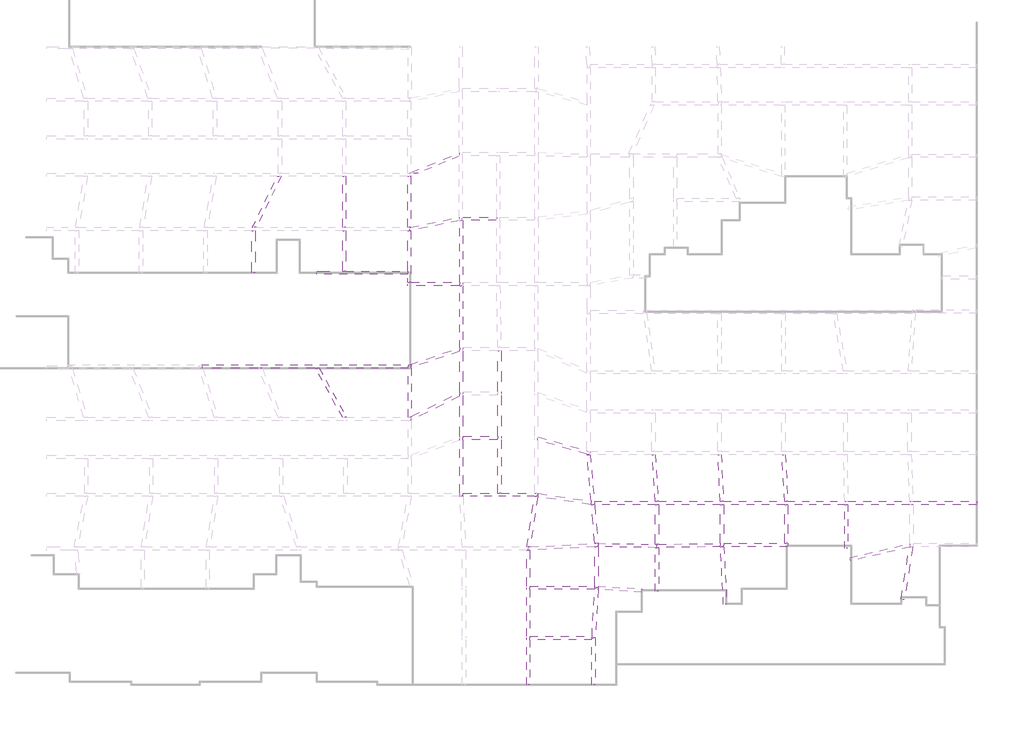
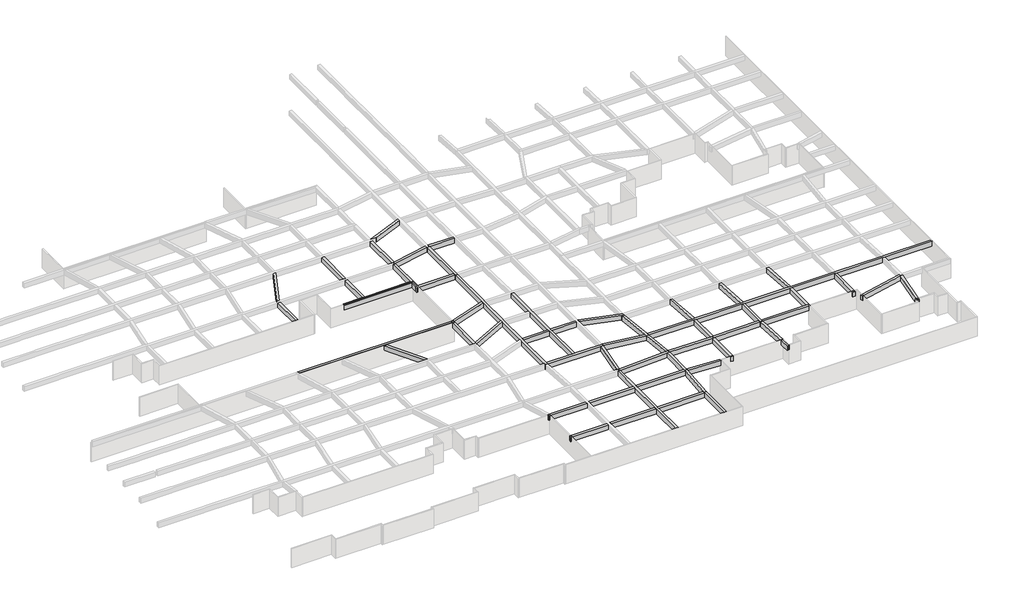
# One storey, part 12 of 45: 49 beams.
# Revit data of these elements (continued)
# Elements 1, 2, 3, 4, 5, 6, 7, 8, 9, 10, 11, 12, 13, 14, 15, 16, 17, 18, 19, 20, 21, 22, 23, 24, 25, 26, 27, 28, 29, 30, 31, 32, 33, 34, 35, 36, 37, 38, 39, 40, 41, 42, 43, 44, 45, 46, 47, 48, 49 (IfcBeam, "混凝土 - 矩形梁 : KL_beam") (continued)
#   Comments = ""
#   Structural Material = none
#   Phase Created = 新构造
# Materials
#   "混凝土 - 现场浇注混凝土": class "混凝土", colour RGB 192 192 192, transparency 0
